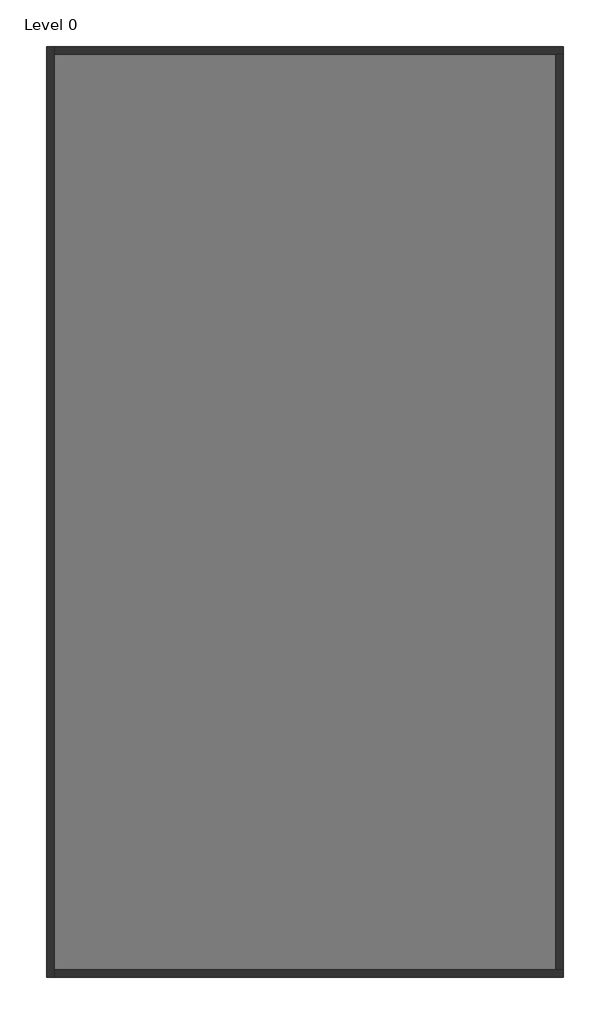
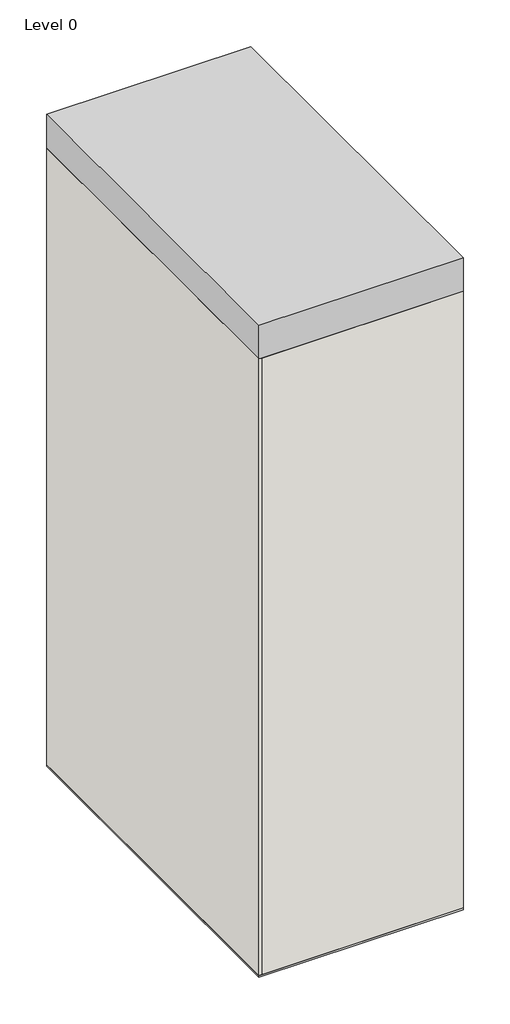
# One storey: 4 walls, 1 proxy, 1 slab.
"""IFC4 building model written with IfcOpenShell, lengths in millimetres."""

from ifc_helpers import new_model, si_unit, frame, origin, origin_with_axes, place, context, project, spatial, polyline, outline, extrude, faceted_brep, element, save

model = new_model("IFC4")

# Units and contexts
model_context = context("Model", 3, world=origin())
ifc_project = project(units=[si_unit("LENGTHUNIT", "METRE", prefix="MILLI")], contexts=[model_context])

# Site, building, storey
site = spatial("IfcSite", under=ifc_project)
building = spatial("IfcBuilding", under=site)
storey = spatial("IfcBuildingStorey", under=building, Name="Level 0", Elevation=100.0)

# Proxy
placement = place(None, origin())
element("IfcBuildingElementProxy", 1, Name="LowUrbanDensityBuilding : LowUrbanDensityBuilding", ObjectType="LowUrbanDensityBuilding : LowUrbanDensityBuilding", at=placement, inside=storey, context=model_context, shape_type="SweptSolid", body=[
    extrude(outline(polyline([(7325.2659446, 3676.2074539), (7325.2659446, -14323.7925461), (-2674.7340554, -14323.7925461), (-2674.7340554, 3676.2074539), (7325.2659446, 3676.2074539)])), origin_with_axes(), (0.0, 0.0, 1.0), 33749.8),
])

# Slab
element("IfcSlab", 2, ObjectType="Floor-Concrete_100Con", at=placement, inside=storey, context=model_context, shape_type="SweptSolid", body=[
    extrude(outline(polyline([(7325.2659446, 3676.2074539), (7325.2659446, -14323.7925461), (-2674.7340554, -14323.7925461), (-2674.7340554, 3676.2074539), (7325.2659446, 3676.2074539)])), origin_with_axes(), (0.0, 0.0, 1.0), 100.0),
])

# Walls
element("IfcWall", 3, ObjectType="Wall-Ext_25Rdr-100Blk-19P", at=placement, inside=storey, context=model_context, shape_type="Brep", body=[
    faceted_brep([(-2674.7340554, 3676.2074539, 100.0), (-2674.7340554, -14323.7925461, 100.0), (-2674.7340554, -14323.7925461, 32000.0), (-2674.7340554, 3676.2074539, 32000.0), (-2530.4340554, 3676.2074539, 100.0), (-2530.4340554, 3676.2074539, 32000.0), (-2530.4340554, 3531.9074539, 32000.0), (-2530.4340554, -14179.4925461, 32000.0), (-2530.4340554, -14323.7925461, 32000.0), (-2530.4340554, -14323.7925461, 100.0), (-2530.4340554, -14179.4925461, 100.0), (-2530.4340554, 3531.9074539, 100.0)], [[[0, 1, 2, 3]], [[4, 5, 6, 7, 8, 9, 10, 11]], [[1, 0, 4, 11, 10, 9]], [[3, 2, 8, 7, 6, 5]], [[2, 1, 9, 8]], [[0, 3, 5, 4]]]),
])
element("IfcWall", 4, ObjectType="Wall-Ext_25Rdr-100Blk-19P", at=placement, inside=storey, context=model_context, shape_type="Brep", body=[
    faceted_brep([(-2530.4340554, -14323.7925461, 100.0), (7325.2659446, -14323.7925461, 100.0), (7325.2659446, -14323.7925461, 32000.0), (-2530.4340554, -14323.7925461, 32000.0), (-2530.4340554, -14179.4925461, 100.0), (-2530.4340554, -14179.4925461, 32000.0), (7180.9659446, -14179.4925461, 32000.0), (7325.2659446, -14179.4925461, 32000.0), (7325.2659446, -14179.4925461, 100.0), (7180.9659446, -14179.4925461, 100.0)], [[[0, 1, 2, 3]], [[4, 5, 6, 7, 8, 9]], [[1, 0, 4, 9, 8]], [[3, 2, 7, 6, 5]], [[0, 3, 5, 4]], [[2, 1, 8, 7]]]),
])
element("IfcWall", 5, ObjectType="Wall-Ext_25Rdr-100Blk-19P", at=placement, inside=storey, context=model_context, shape_type="Brep", body=[
    faceted_brep([(7325.2659446, 3676.2074539, 100.0), (-2530.4340554, 3676.2074539, 100.0), (-2530.4340554, 3676.2074539, 32000.0), (7325.2659446, 3676.2074539, 32000.0), (7325.2659446, 3531.9074539, 100.0), (7325.2659446, 3531.9074539, 32000.0), (7180.9659446, 3531.9074539, 32000.0), (-2530.4340554, 3531.9074539, 32000.0), (-2530.4340554, 3531.9074539, 100.0), (7180.9659446, 3531.9074539, 100.0)], [[[0, 1, 2, 3]], [[4, 5, 6, 7, 8, 9]], [[1, 0, 4, 9, 8]], [[3, 2, 7, 6, 5]], [[2, 1, 8, 7]], [[0, 3, 5, 4]]]),
])
element("IfcWall", 6, ObjectType="Wall-Ext_25Rdr-100Blk-19P", at=placement, inside=storey, context=model_context, shape_type="SweptSolid", body=[
    extrude(outline(polyline([(7325.2659446, 3531.9074539), (7325.2659446, -14179.4925461), (7180.9659446, -14179.4925461), (7180.9659446, 3531.9074539), (7325.2659446, 3531.9074539)])), frame((0.0, 0.0, 100.0), z_axis=(0.0, 0.0, 1.0), x_axis=(1.0, 0.0, 0.0)), (0.0, 0.0, 1.0), 31900.0),
])

save(model, "model.ifc")

# Revit data of these elements
# Project information
#   Project Issue Date = "Issue Date"
#   Project Status = "Project Status"
#   Client Name = "Owner"
#   Project Address = "Enter address here"
#   Project Name = "Project Name"
#   Project Number = "Project Number"
# Type "Floor-Concrete_100Con"
#   Keynote = "E60/130"
#   Function = 0
#   Layers, outside or top first: 100 mm "Concrete" (function 1)
# Type "Wall-Ext_25Rdr-100Blk-19P"
#   Keynote = "F10"
#   Layers, outside or top first: 25.3 mm "Render, Beige, Smooth" (function 5); 100 mm "Concrete Masonry Units _Low Density" (function 1); 19 mm "Plaster" (function 5)
# Element 1 (IfcBuildingElementProxy, "LowUrbanDensityBuilding : LowUrbanDensityBuilding")
#   Phase Created = New Construction
#   Materials on its faces: "Default Form"
# Element 2 (IfcSlab, "Floor-Concrete_100Con")
#   Height Offset From Level = 0 mm
#   Phase Created = New Construction
#   Materials on its faces: "Concrete"
# Element 3 (IfcWall, "Wall-Ext_25Rdr-100Blk-19P")
#   Top Offset = 0 mm
#   Base Offset = 0 mm
#   wall height = 31900 mm
#   Phase Created = New Construction
#   Base Constraint = Level 0
#   Top Constraint = Level 8
#   Materials on its faces: "Render, Beige, Smooth", "Default Wall", "Plaster"
# Elements 4, 5, 6 (IfcWall, "Wall-Ext_25Rdr-100Blk-19P")
#   Top Offset = 0 mm
#   Base Offset = 0 mm
#   wall height = 31900 mm
#   Phase Created = New Construction
#   Base Constraint = Level 0
#   Top Constraint = Level 8
#   Materials on its faces: "Default Wall", "Render, Beige, Smooth", "Plaster"
# Materials
#   "Concrete": class "Concrete", colour RGB 120 120 120, transparency 0, Description = "Portland Cement Concrete", Cost = 0
#   "Render, Beige, Smooth": class "Generic", colour RGB 213 198 180, transparency 0, Description = "physical material", Cost = 0
#   "Concrete Masonry Units _Low Density": class "Masonry", colour RGB 181 181 181, transparency 0, Description = "Concrete masonry units", Cost = 0
#   "Plaster": class "Generic", colour RGB 249 249 249, transparency 0, Description = "Plaster", Cost = 0
#   "Default Form": class "Generic", colour RGB 185 189 196, transparency 0.5, Cost = 0
#   "Default Wall": class "Miscellaneous", colour RGB 128 128 128, transparency 0, Comments = "Rendering appearance not upgraded Rendering appearance not upgraded ", Cost = 0
